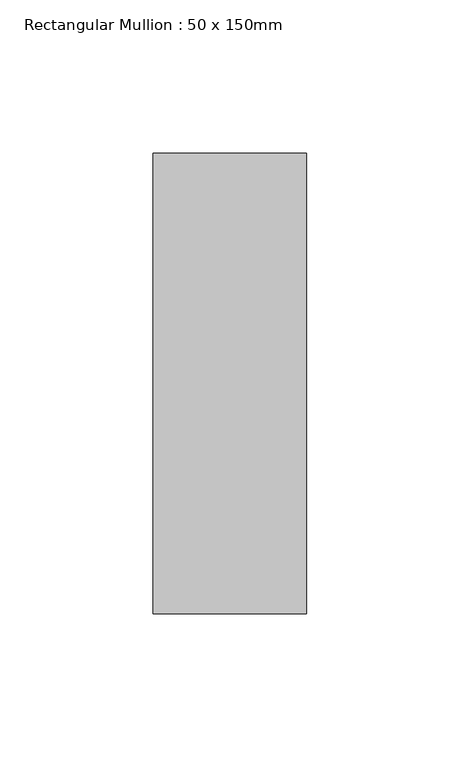
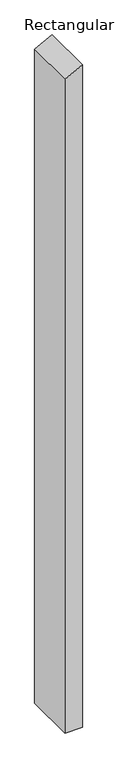
"""IFC4 building model written with IfcOpenShell, lengths in millimetres: member geometry, Rectangular Mullion : 50 x 150mm."""

from ifc_helpers import new_model, si_unit, frame, origin, place, context, project, spatial, polyline, outline, extrude, source, transform, mapped, element, save


def rectangular_mullion_50_x_150mm_b54f717a(model_context):
    return source(origin(), model_context, "Body", "SweptSolid", [
        extrude(outline(polyline([(0.0, 0.0), (-26.0283525, -50.0), (-2010.0622615, -50.0), (-2010.0622615, 0.0), (0.0, 0.0)])), frame((0.0, -75.0, 0.0), z_axis=(0.0, 1.0, 0.0), x_axis=(0.0, 0.0, 1.0)), (0.0, 0.0, 1.0), 150.0),
    ])


if __name__ == "__main__":
    model = new_model("IFC4")
    model_context = context("Model", 3, world=origin())
    ifc_project = project(units=[si_unit("LENGTHUNIT", "METRE", prefix="MILLI")], contexts=[model_context])
    site = spatial("IfcSite", under=ifc_project)
    building = spatial("IfcBuilding", under=site)
    placement = place(None, origin())
    rectangular_mullion_50_x_150mm_shape = rectangular_mullion_50_x_150mm_b54f717a(model_context)
    element("IfcMember", 1, ObjectType="Rectangular Mullion : 50 x 150mm", at=placement, inside=building, context=model_context, shape_type="MappedRepresentation", body=[
        mapped(rectangular_mullion_50_x_150mm_shape, transform((0.0, 0.0, 0.0), x_axis=(1.0, 0.0, 0.0), y_axis=(0.0, 1.0, 0.0), z_axis=(0.0, 0.0, 1.0))),
    ])
    save(model, "model.ifc")

# Revit data of these elements
# Type "Rectangular Mullion : 50 x 150mm"
#   built-in parameter 1007304 = 0.492126 (stored number, unit not read)
#   built-in parameter 1007301 = 0.082021 (stored number, unit not read)
#   built-in parameter 1007300 = 0.082021 (stored number, unit not read)
# Element 1 (IfcMember, "Rectangular Mullion : 50 x 150mm")
#   Materials on its faces: "Aluminium"
# Materials
#   "Aluminium": class "Metal", colour RGB 247 247 247, transparency 0, Description = "Aluminium 6061", Cost = 0
